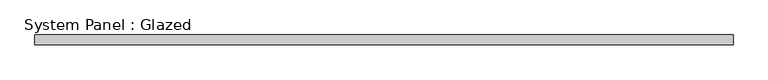
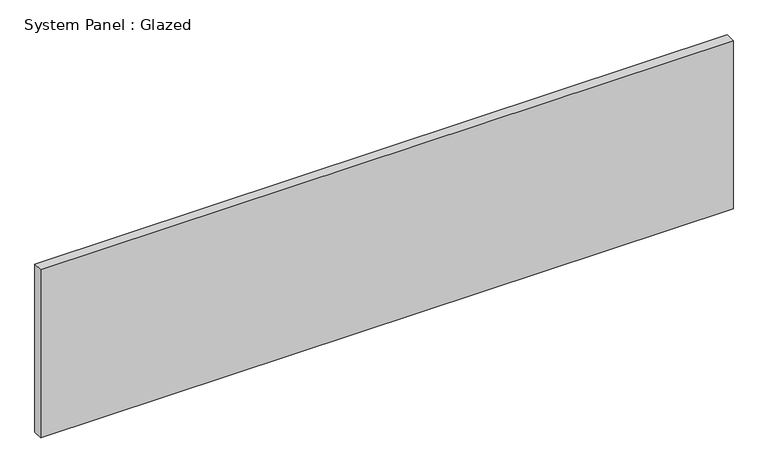
"""IFC4 building model written with IfcOpenShell, lengths in millimetres: plate geometry, System Panel : Glazed."""

from ifc_helpers import new_model, si_unit, origin, origin_with_axes, place, context, project, spatial, polyline, outline, extrude, source, transform, mapped, element, save


def system_panel_glazed_b225d226(model_context):
    return source(origin(), model_context, "Body", "SweptSolid", [
        extrude(outline(polyline([(877.5, 24.5), (-877.5, 24.5), (-877.5, 49.5), (877.5, 49.5), (877.5, 24.5)])), origin_with_axes(), (0.0, 0.0, 1.0), 450.0),
    ])


if __name__ == "__main__":
    model = new_model("IFC4")
    model_context = context("Model", 3, world=origin())
    ifc_project = project(units=[si_unit("LENGTHUNIT", "METRE", prefix="MILLI")], contexts=[model_context])
    site = spatial("IfcSite", under=ifc_project)
    building = spatial("IfcBuilding", under=site)
    placement = place(None, origin())
    system_panel_glazed_shape = system_panel_glazed_b225d226(model_context)
    element("IfcPlate", 1, ObjectType="System Panel : Glazed", at=placement, inside=building, context=model_context, shape_type="MappedRepresentation", body=[
        mapped(system_panel_glazed_shape, transform((0.0, 0.0, 0.0), x_axis=(1.0, 0.0, 0.0), y_axis=(0.0, 1.0, 0.0), z_axis=(0.0, 0.0, 1.0))),
    ])
    save(model, "model.ifc")

# Revit data of these elements
# Type "System Panel : Glazed"
#   Keynote = "H11"
#   Construction Type Id = "GSP4R"
#   Analytic Construction = "1/8 in Pilkington single glazing"
#   Visual Light Transmittance = 0.9
#   Solar Heat Gain Coefficient = 0.86
#   Heat Transfer Coefficient (U) = 6.7069 W/(m²·K)
# Element 1 (IfcPlate, "System Panel : Glazed")
#   Materials on its faces: "Glass"
# Materials
#   "Glass": class "Glass", colour RGB 0 128 192, transparency 0.9, Description = "Soda Lime Glass", Cost = 0
